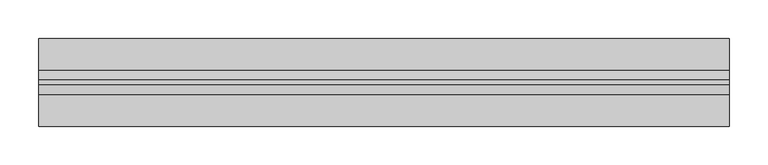
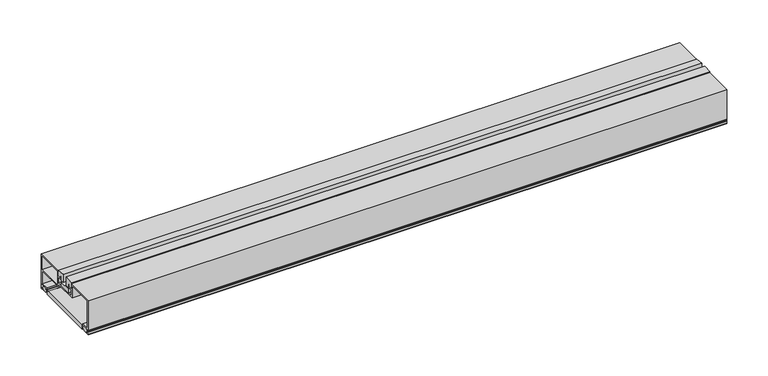
"""IFC4 building model written with IfcOpenShell, lengths in millimetres: proxy geometry, Generic Models 3:Generic Models 1:2:Generic Models 1:2 : Generic Models 3:Generic Models 1:300625:328150:Generic Models 1:2:Generic Models 1:2 : Generic Models 3:Generic Models 1:300625:328150 : Generic Models 3:Generic Models 1:2:Generic Models 1:2 : Generic Models 3:Generic Models 1:300625:328150:3 : Generic Models 3:Generic Models 1:2:Generic Models 1:2 : Generic Models 3:Generic Models 1:300625:328150:Generic Models 1:2:Generic Models 1:2 : Generic Models 3:Generic Models 1:300625:328150 : Generic Models 3:Generic Models 1:2:Generic Models 1:2 : Generic Models 3:Generic Models 1:300625:328150:300962."""

from ifc_helpers import new_model, si_unit, frame, origin, place, context, project, spatial, polyline, outline, extrude, source, transform, mapped, element, save


def generic_models_21ac7cc4(model_context):
    return source(origin(), model_context, "Body", "SweptSolid", [
        extrude(outline(polyline([(-568050.8100714, 46.8872108), (-568050.8100714, 41.1736702), (-568055.5641272, 41.1736702), (-568055.5641272, 53.2439273), (-568043.6663214, 51.7830605), (-568043.6663214, 43.9433511), (-568047.9643932, 43.9433511), (-568047.9643932, 46.8872108), (-568050.8100714, 46.8872108)])), frame((592836.3867242, 0.0, 0.0), z_axis=(1.0, 0.0, 0.0), x_axis=(0.0, 1.0, 0.0)), (0.0, 0.0, 1.0), 895.35),
        extrude(outline(polyline([(593731.7367242, -568016.9406051), (593731.7367242, -568102.342163), (592836.3867242, -568102.342163), (592836.3867242, -568016.9406051), (593731.7367242, -568016.9406051)])), frame((0.0, 0.0, 0.0018625), z_axis=(0.0, 0.0, 1.0), x_axis=(1.0, 0.0, 0.0)), (0.0, 0.0, 1.0), 6.35),
        extrude(outline(polyline([(-568002.371855, 5.3860992), (-568002.6855411, 3.1768625), (-568002.371855, 0.9676257), (-568001.9944464, 0.0018625), (-568007.8625385, 0.0018625), (-568007.0022575, 0.38818), (-568005.6926824, 1.4716655), (-568005.0923289, 2.8219132), (-568005.2951168, 4.2276895), (-568006.2693218, 5.4690736), (-568007.8625385, 6.3518625), (-568001.9944464, 6.3518625), (-568002.371855, 5.3860992)])), frame((592836.3867242, 0.0, 0.0), z_axis=(1.0, 0.0, 0.0), x_axis=(0.0, 1.0, 0.0)), (0.0, 0.0, 1.0), 895.35),
        extrude(outline(polyline([(-568005.9353019, 1.7992816), (-568007.2567959, 0.6945475), (-568009.1664101, 0.0814663), (-568010.2261661, 0.0018625), (-568011.285922, 0.0814663), (-568013.1955363, 0.6945475), (-568014.5170303, 1.7992816), (-568014.9886661, 3.1768625), (-568014.5170303, 4.5544433), (-568013.1955363, 5.6591774), (-568011.285922, 6.2722586), (-568010.2261661, 6.3518625), (-568009.1664101, 6.2722586), (-568007.2567959, 5.6591774), (-568005.9353019, 4.5544433), (-568005.4636661, 3.1768625), (-568005.9353019, 1.7992816)])), frame((592836.3867242, 0.0, 0.0), z_axis=(1.0, 0.0, 0.0), x_axis=(0.0, 1.0, 0.0)), (0.0, 0.0, 1.0), 895.35),
        extrude(outline(polyline([(-568107.0029708, 0.0814663), (-568108.0627267, 0.0018625), (-568109.1224826, 0.0814663), (-568111.0320969, 0.6945475), (-568112.3535909, 1.7992816), (-568112.8252267, 3.1768625), (-568112.3535909, 4.5544433), (-568111.0320969, 5.6591774), (-568109.1224826, 6.2722586), (-568108.0627267, 6.3518625), (-568107.0029708, 6.2722586), (-568105.0933565, 5.6591774), (-568103.7718625, 4.5544433), (-568103.3002267, 3.1768625), (-568103.7718625, 1.7992816), (-568105.0933565, 0.6945475), (-568107.0029708, 0.0814663)])), frame((592836.3867242, 0.0, 0.0), z_axis=(1.0, 0.0, 0.0), x_axis=(0.0, 1.0, 0.0)), (0.0, 0.0, 1.0), 895.35),
        extrude(outline(polyline([(-568110.4263543, 0.0018625), (-568116.2944464, 0.0018625), (-568115.9170378, 0.9676257), (-568115.6033517, 3.1768625), (-568115.9170378, 5.3860992), (-568116.2944464, 6.3518625), (-568110.4263543, 6.3518625), (-568112.019571, 5.4690736), (-568112.993776, 4.2276895), (-568113.1965639, 2.8219132), (-568112.5962104, 1.4716655), (-568111.2866352, 0.38818), (-568110.4263543, 0.0018625)])), frame((592836.3867242, 0.0, 0.0), z_axis=(1.0, 0.0, 0.0), x_axis=(0.0, 1.0, 0.0)), (0.0, 0.0, 1.0), 895.35),
        extrude(outline(polyline([(593731.7367242, -568050.8100714), (593731.7367242, -568067.4788214), (592836.3867242, -568067.4788214), (592836.3867242, -568050.8100714), (593731.7367242, -568050.8100714)])), frame((0.0, 0.0, 32.9494693), z_axis=(0.0, 0.0, 1.0), x_axis=(1.0, 0.0, 0.0)), (0.0, 0.0, 1.0), 5.5626),
        extrude(outline(polyline([(-568067.4788214, 46.8872108), (-568070.3244996, 46.8872108), (-568070.3244996, 43.9433511), (-568074.6225714, 43.9433511), (-568074.6225714, 51.7830605), (-568062.7247655, 53.2439273), (-568062.7247655, 41.1736702), (-568067.4788214, 41.1736702), (-568067.4788214, 46.8872108)])), frame((592836.3867242, 0.0, 0.0), z_axis=(1.0, 0.0, 0.0), x_axis=(0.0, 1.0, 0.0)), (0.0, 0.0, 1.0), 895.35),
        extrude(outline(polyline([(-568116.2944464, 6.35), (-568116.2944464, 50.7662234), (-568074.9780601, 50.7662234), (-568074.9780601, 43.5464761), (-568069.8862383, 43.5464761), (-568069.8862383, 46.4903358), (-568067.8343101, 46.4903358), (-568067.8343101, 41.5705452), (-568074.9780601, 41.5705452), (-568074.9780601, 32.9494693), (-568043.3108327, 32.9494693), (-568043.3108327, 41.5705452), (-568050.4545827, 41.5705452), (-568050.4545827, 46.4903358), (-568048.4026545, 46.4903358), (-568048.4026545, 43.5464761), (-568043.3108327, 43.5464761), (-568043.3108327, 50.7662234), (-568001.9944464, 50.7662234), (-568001.9944464, 6.35), (-568015.0815775, 6.35), (-568015.0815775, 8.2499335), (-568004.5023586, 8.2499335), (-568004.5023586, 27.4630693), (-568043.3108327, 27.4630693), (-568043.3108327, 31.0495358), (-568076.8779936, 31.0495358), (-568076.8779936, 48.8662899), (-568113.7865342, 48.8662899), (-568113.7865342, 8.2499335), (-568103.2073153, 8.2499335), (-568103.2073153, 6.35), (-568116.2944464, 6.35)]), holes=[polyline([(-568041.4108992, 29.3630028), (-568004.5023586, 29.3630028), (-568004.5023586, 48.8662899), (-568041.4108992, 48.8662899), (-568041.4108992, 29.3630028)])]), frame((592836.3867242, 0.0, 0.0), z_axis=(1.0, 0.0, 0.0), x_axis=(0.0, 1.0, 0.0)), (0.0, 0.0, 1.0), 895.35),
    ])


if __name__ == "__main__":
    model = new_model("IFC4")
    model_context = context("Model", 3, world=origin())
    ifc_project = project(units=[si_unit("LENGTHUNIT", "METRE", prefix="MILLI")], contexts=[model_context])
    site = spatial("IfcSite", under=ifc_project)
    building = spatial("IfcBuilding", under=site)
    placement = place(None, origin())
    generic_models_shape = generic_models_21ac7cc4(model_context)
    element("IfcBuildingElementProxy", 1, Name="Generic Models 3:Generic Models 1:2:Generic Models 1:2 : Generic Models 3:Generic Models 1:300625:328150:Generic Models 1:2:Generic Models 1:2 : Generic Models 3:Generic Models 1:300625:328150 : Generic Models 3:Generic Models 1:2:Generic Models 1:2 : Generic Models 3:Generic Models 1:300625:328150:3 : Generic Models 3:Generic Models 1:2:Generic Models 1:2 : Generic Models 3:Generic Models 1:300625:328150:Generic Models 1:2:Generic Models 1:2 : Generic Models 3:Generic Models 1:300625:328150 : Generic Models 3:Generic Models 1:2:Generic Models 1:2 : Generic Models 3:Generic Models 1:300625:328150:300962", ObjectType="Generic Models 3:Generic Models 1:2:Generic Models 1:2 : Generic Models 3:Generic Models 1:300625:328150:Generic Models 1:2:Generic Models 1:2 : Generic Models 3:Generic Models 1:300625:328150 : Generic Models 3:Generic Models 1:2:Generic Models 1:2 : Generic Models 3:Generic Models 1:300625:328150:3 : Generic Models 3:Generic Models 1:2:Generic Models 1:2 : Generic Models 3:Generic Models 1:300625:328150:Generic Models 1:2:Generic Models 1:2 : Generic Models 3:Generic Models 1:300625:328150 : Generic Models 3:Generic Models 1:2:Generic Models 1:2 : Generic Models 3:Generic Models 1:300625:328150:300962", at=placement, inside=building, context=model_context, shape_type="MappedRepresentation", body=[
        mapped(generic_models_shape, transform((0.0, 0.0, 0.0), x_axis=(1.0, 0.0, 0.0), y_axis=(0.0, 1.0, 0.0), z_axis=(0.0, 0.0, 1.0))),
    ])
    save(model, "model.ifc")

# Revit data of these elements
# Type "Generic Models 3:Generic Models 1:2:Generic Models 1:2 : Generic Models 3:Generic Models 1:300625:328150:Generic Models 1:2:Generic Models 1:2 : Generic Models 3:Generic Models 1:300625:328150 : Generic Models 3:Generic Models 1:2:Generic Models 1:2 : Generic Models 3:Generic Models 1:300625:328150:3 : Generic Models 3:Generic Models 1:2:Generic Models 1:2 : Generic Models 3:Generic Models 1:300625:328150:Generic Models 1:2:Generic Models 1:2 : Generic Models 3:Generic Models 1:300625:328150 : Generic Models 3:Generic Models 1:2:Generic Models 1:2 : Generic Models 3:Generic Models 1:300625:328150:300962"
#   NameOverride = "Generic Models 3:Generic Models 1:2:Generic Models 1:2 : Generic Models 3:Generic Models 1:300625:328150:Generic Models 1:2:Generic Models 1:2 : Generic Models 3:Generic Models 1:300625:328150 : Generic Models 3:Generic Models 1:2:Generic Models 1:2 : Generic Models 3:Generic Models 1:300625:328150:300962"
#   ObjectTypeOverride = "Generic Models 1:2:Generic Models 1:2 : Generic Models 3:Generic Models 1:300625:328150 : Generic Models 3:Generic Models 1:2:Generic Models 1:2 : Generic Models 3:Generic Models 1:300625:328150"
#   Reference = "Generic Models 1"
#   Tag = "300962"
# Element 1 (IfcBuildingElementProxy, "Generic Models 3:Generic Models 1:2:Generic Models 1:2 : Generic Models 3:Generic Models 1:300625:328150:Generic Models 1:2:Generic Models 1:2 : Generic Models 3:Generic Models 1:300625:328150 : Generic Models 3:Generic Models 1:2:Generic Models 1:2 : Generic Models 3:Generic Models 1:300625:328150:3 : Generic Models 3:Generic Models 1:2:Generic Models 1:2 : Generic Models 3:Generic Models 1:300625:328150:Generic Models 1:2:Generic Models 1:2 : Generic Models 3:Generic Models 1:300625:328150 : Generic Models 3:Generic Models 1:2:Generic Models 1:2 : Generic Models 3:Generic Models 1:300625:328150:300962")
#   Materials on its faces: "SEALANT & BACKER ROD, IF NECESSARY", "INTERIOR GRADE ALUMINUM STOREFRONT W/ SINGLE GLAZING"
# Materials
#   "SEALANT & BACKER ROD, IF NECESSARY": class "Unassigned", colour RGB 120 120 120, transparency 0, Cost = 0
#   "INTERIOR GRADE ALUMINUM STOREFRONT W/ SINGLE GLAZING": class "Unassigned", colour RGB 244 244 244, transparency 0, Cost = 0
